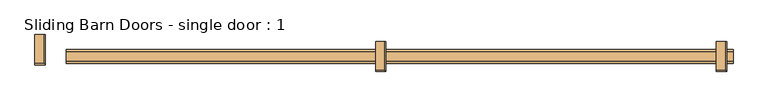
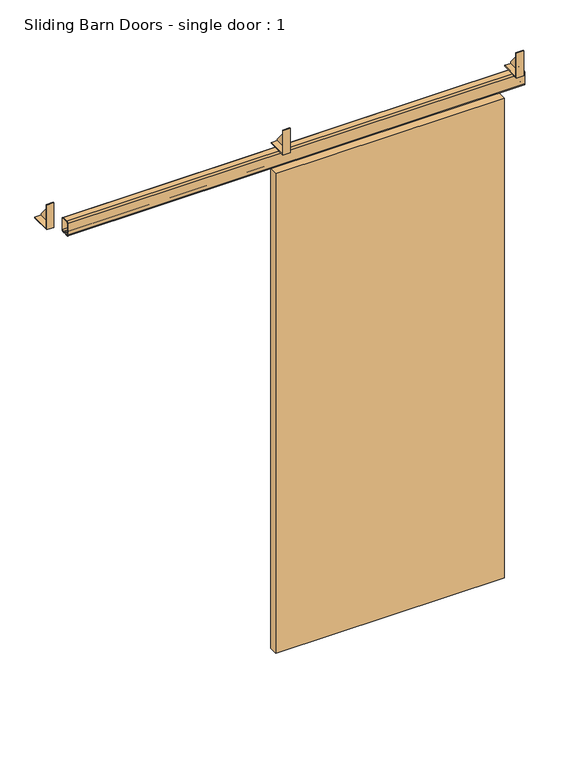
"""IFC4 building model written with IfcOpenShell, lengths in millimetres: door geometry, Sliding Barn Doors - single door : 1."""

from ifc_helpers import new_model, si_unit, point, frame, frame_2d, origin, place, context, project, spatial, polyline, circle_curve, trimmed, segment, composite_curve, outline, extrude, source, transform, mapped, element, save


def sliding_barn_doors_single_door_1_d957e45b(model_context):
    return source(origin(), model_context, "Body", "SweptSolid", [
        extrude(outline(polyline([(158.75, 2152.65), (158.75, 2146.3), (79.375, 2146.3), (79.375, 2247.773), (158.75, 2152.65)])), frame((-1418.4808594, 0.0, 0.0), z_axis=(1.0, 0.0, 0.0), x_axis=(0.0, 1.0, 0.0)), (0.0, 0.0, 1.0), 3.175),
        extrude(outline(polyline([(76.2, 2143.125), (76.2, 2247.773), (79.375, 2247.773), (79.375, 2146.3), (158.75, 2146.3), (158.75, 2143.125), (76.2, 2143.125)])), frame((-1443.7816406, 0.0, 0.0), z_axis=(1.0, 0.0, 0.0), x_axis=(0.0, 1.0, 0.0)), (0.0, 0.0, 1.0), 28.4757812),
        extrude(outline(polyline([(139.7, 2152.65), (139.7, 2146.3), (60.325, 2146.3), (60.325, 2247.773), (139.7, 2152.65)])), frame((-484.2371094, 0.0, 0.0), z_axis=(1.0, 0.0, 0.0), x_axis=(0.0, 1.0, 0.0)), (0.0, 0.0, 1.0), 3.175),
        extrude(outline(polyline([(57.15, 2143.125), (57.15, 2247.773), (60.325, 2247.773), (60.325, 2146.3), (139.7, 2146.3), (139.7, 2143.125), (57.15, 2143.125)])), frame((-509.5378906, 0.0, 0.0), z_axis=(1.0, 0.0, 0.0), x_axis=(0.0, 1.0, 0.0)), (0.0, 0.0, 1.0), 28.4757813),
        extrude(outline(polyline([(139.7, 2152.65), (139.7, 2146.3), (60.325, 2146.3), (60.325, 2247.773), (139.7, 2152.65)])), frame((450.0066406, 0.0, 0.0), z_axis=(1.0, 0.0, 0.0), x_axis=(0.0, 1.0, 0.0)), (0.0, 0.0, 1.0), 3.175),
        extrude(outline(polyline([(57.15, 2143.125), (57.15, 2247.773), (60.325, 2247.773), (60.325, 2146.3), (139.7, 2146.3), (139.7, 2143.125), (57.15, 2143.125)])), frame((424.7058594, 0.0, 0.0), z_axis=(1.0, 0.0, 0.0), x_axis=(0.0, 1.0, 0.0)), (0.0, 0.0, 1.0), 28.4757813),
        extrude(outline(polyline([(-424.91025, 117.475), (-373.60225, 117.475), (-373.60225, 114.3), (-424.91025, 114.3), (-424.91025, 117.475)])), frame((0.0, 0.0, 1889.252), z_axis=(0.0, 0.0, 1.0), x_axis=(1.0, 0.0, 0.0)), (0.0, 0.0, 1.0), 168.148),
        extrude(outline(polyline([(235.48975, 117.475), (286.79775, 117.475), (286.79775, 114.3), (235.48975, 114.3), (235.48975, 117.475)])), frame((0.0, 0.0, 1889.252), z_axis=(0.0, 0.0, 1.0), x_axis=(1.0, 0.0, 0.0)), (0.0, 0.0, 1.0), 168.148),
        extrude(outline(polyline([(-526.25625, 114.3), (388.14375, 114.3), (388.14375, 79.375), (-526.25625, 79.375), (-526.25625, 114.3)])), frame((0.0, 0.0, 25.4), z_axis=(0.0, 0.0, 1.0), x_axis=(1.0, 0.0, 0.0)), (0.0, 0.0, 1.0), 2032.0),
        extrude(outline(composite_curve([segment(polyline([(85.725, 2143.125), (111.252, 2143.125)]), True, "CONTINUOUS"), segment(trimmed(circle_curve(frame_2d((111.252, 2136.775)), 6.35), [point((111.252, 2143.125))], [point((117.602, 2136.775))], False, "CARTESIAN"), True, "CONTINUOUS"), segment(polyline([(117.602, 2136.775), (117.602, 2088.515)]), True, "CONTINUOUS"), segment(trimmed(circle_curve(frame_2d((111.252, 2088.515)), 6.35), [point((117.602, 2088.515))], [point((111.252, 2082.165))], False, "CARTESIAN"), True, "CONTINUOUS"), segment(polyline([(111.252, 2082.165), (105.8433147, 2082.165)]), True, "CONTINUOUS"), segment(trimmed(circle_curve(frame_2d((105.8433147, 2083.7525)), 1.5875), [point((105.8433147, 2082.165))], [point((104.2849816, 2083.4495907))], False, "CARTESIAN"), True, "CONTINUOUS"), segment(polyline([(104.2849816, 2083.4495907), (102.8594659, 2090.7832331), (104.3756029, 2090.7832331), (105.7615251, 2083.6532812), (111.252, 2083.6532812)]), True, "CONTINUOUS"), segment(trimmed(circle_curve(frame_2d((111.252, 2088.515)), 4.8617187), [point((111.252, 2083.6532812))], [point((116.1137188, 2088.515))], True, "CARTESIAN"), True, "CONTINUOUS"), segment(polyline([(116.1137188, 2088.515), (116.1137188, 2136.775)]), True, "CONTINUOUS"), segment(trimmed(circle_curve(frame_2d((111.252, 2136.775)), 4.8617187), [point((116.1137188, 2136.775))], [point((111.252, 2141.6367187))], True, "CARTESIAN"), True, "CONTINUOUS"), segment(polyline([(111.252, 2141.6367187), (85.725, 2141.6367187)]), True, "CONTINUOUS"), segment(trimmed(circle_curve(frame_2d((85.725, 2136.775)), 4.8617187), [point((85.725, 2141.6367187))], [point((80.8632813, 2136.775))], True, "CARTESIAN"), True, "CONTINUOUS"), segment(polyline([(80.8632813, 2136.775), (80.8632813, 2088.515)]), True, "CONTINUOUS"), segment(trimmed(circle_curve(frame_2d((85.725, 2088.515)), 4.8617187), [point((80.8632813, 2088.515))], [point((85.725, 2083.6532812))], True, "CARTESIAN"), True, "CONTINUOUS"), segment(polyline([(85.725, 2083.6532812), (91.2154749, 2083.6532812), (92.6013971, 2090.7832331), (94.1175341, 2090.7832331), (92.6920184, 2083.4495907)]), True, "CONTINUOUS"), segment(trimmed(circle_curve(frame_2d((91.1336853, 2083.7525)), 1.5875), [point((92.6920184, 2083.4495907))], [point((91.1336853, 2082.165))], False, "CARTESIAN"), True, "CONTINUOUS"), segment(polyline([(91.1336853, 2082.165), (85.725, 2082.165)]), True, "CONTINUOUS"), segment(trimmed(circle_curve(frame_2d((85.725, 2088.515)), 6.35), [point((85.725, 2082.165))], [point((79.375, 2088.515))], False, "CARTESIAN"), True, "CONTINUOUS"), segment(polyline([(79.375, 2088.515), (79.375, 2136.775)]), True, "CONTINUOUS"), segment(trimmed(circle_curve(frame_2d((85.725, 2136.775)), 6.35), [point((79.375, 2136.775))], [point((85.725, 2143.125))], False, "CARTESIAN"), True, "CONTINUOUS")], self_intersect=False)), frame((-1358.10625, 0.0, 0.0), z_axis=(1.0, 0.0, 0.0), x_axis=(0.0, 1.0, 0.0)), (0.0, 0.0, 1.0), 1828.8),
    ])


if __name__ == "__main__":
    model = new_model("IFC4")
    model_context = context("Model", 3, world=origin())
    ifc_project = project(units=[si_unit("LENGTHUNIT", "METRE", prefix="MILLI")], contexts=[model_context])
    site = spatial("IfcSite", under=ifc_project)
    building = spatial("IfcBuilding", under=site)
    placement = place(None, origin())
    sliding_barn_doors_single_door_1_shape = sliding_barn_doors_single_door_1_d957e45b(model_context)
    element("IfcDoor", 1, ObjectType="Sliding Barn Doors - single door : 1", at=placement, inside=building, context=model_context, shape_type="MappedRepresentation", body=[
        mapped(sliding_barn_doors_single_door_1_shape, transform((0.0, 0.0, 0.0), x_axis=(1.0, 0.0, 0.0), y_axis=(0.0, 1.0, 0.0), z_axis=(0.0, 0.0, 1.0))),
    ])
    save(model, "model.ifc")

# Revit data of these elements
# Type "Sliding Barn Doors - single door : 1"
#   Type Mark = "61"
#   OD_DS_Door_Material = "T.B.D."
#   OD_DS_Door_Type = "SLIDER"
#   OD_DS_Lockset = "-"
#   Analytic Construction = "<None>"
#   rail_overlap_left = 0' - 5 1/4"
#   rail_length = 6' - 0"
#   overlap_left = 0' - 2"
#   overlap = 0' - 0"
#   bracket_right = 3' - 7"
#   bracket_left = 0' - 4"
#   Thickness = 0' - 1 3/8"
#   Panel Width = 3' - 0"
#   Panel Height = 6' - 8"
#   Gap 2 = 0' - 0 1/2"
#   Gap 1 = 0' - 0 7/8"
#   Frame Projection Ext. = 0' - 1"
#   Frame Projection Int. = 0' - 1"
#   Frame Width = 0' - 3"
#   Height = 6' - 4"
#   Width = 2' - 2 9/16"
#   Bracket_offset = 0' - 5"
#   Door_4 = no
#   Door_3 = no
#   Hardware Material = Metal - Aluminum
#   Door Material = Closet_1
#   Function = (empty or 0)
#   Wall Closure = (empty or 0)
# Element 1 (IfcDoor, "Sliding Barn Doors - single door : 1")
#   Materials on its faces: "Metal - Aluminum", "Closet_1"
# Materials
#   "Metal - Aluminum": class "Metal", colour RGB 247 247 247, transparency 0
#   "Closet_1": class "Paint", colour RGB 200 194 183, transparency 0, Cost = 0
